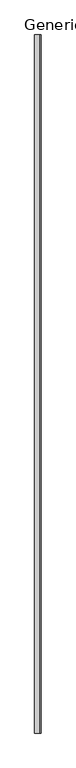
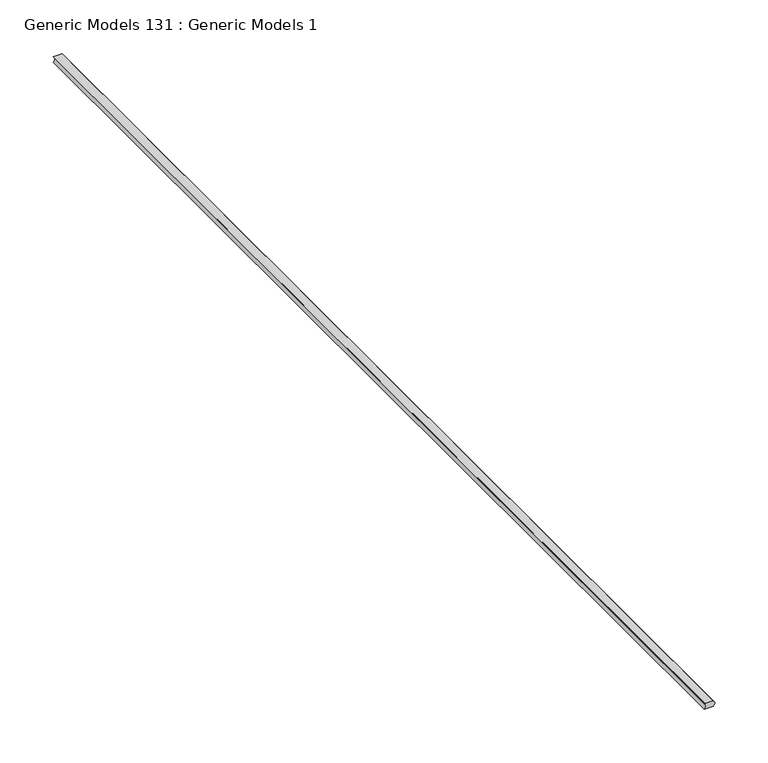
"""IFC4 building model written with IfcOpenShell, lengths in millimetres: proxy geometry, Generic Models 131 : Generic Models 1."""

from ifc_helpers import new_model, si_unit, point, frame, frame_2d, origin, place, context, project, spatial, polyline, circle_curve, trimmed, segment, composite_curve, outline, extrude, source, transform, mapped, element, save


def generic_models_131_generic_models_1_f9918aae(model_context):
    return source(origin(), model_context, "Body", "SweptSolid", [
        extrude(outline(composite_curve([segment(polyline([(0.0, 50777.775), (0.0, 50787.3)]), True, "CONTINUOUS"), segment(trimmed(circle_curve(frame_2d((3.175, 50784.3852595)), 4.3100275), [point((0.0, 50787.3))], [point((6.35, 50787.3))], False, "CARTESIAN"), True, "CONTINUOUS"), segment(polyline([(6.35, 50787.3), (6.35, 50777.775)]), True, "CONTINUOUS"), segment(trimmed(circle_curve(frame_2d((3.175, 50774.8602595)), 4.3100275), [point((6.35, 50777.775))], [point((0.0, 50777.775))], True, "CARTESIAN"), True, "CONTINUOUS")], self_intersect=False)), frame((0.0, 0.0, 0.0), z_axis=(0.0, 1.0, 0.0), x_axis=(0.0, 0.0, 1.0)), (0.0, 0.0, 1.0), 1219.2),
    ])


if __name__ == "__main__":
    model = new_model("IFC4")
    model_context = context("Model", 3, world=origin())
    ifc_project = project(units=[si_unit("LENGTHUNIT", "METRE", prefix="MILLI")], contexts=[model_context])
    site = spatial("IfcSite", under=ifc_project)
    building = spatial("IfcBuilding", under=site)
    placement = place(None, origin())
    generic_models_131_generic_models_1_shape = generic_models_131_generic_models_1_f9918aae(model_context)
    element("IfcBuildingElementProxy", 1, Name="Generic Models 131 : Generic Models 1", ObjectType="Generic Models 131 : Generic Models 1", at=placement, inside=building, context=model_context, shape_type="MappedRepresentation", body=[
        mapped(generic_models_131_generic_models_1_shape, transform((0.0, 0.0, 0.0), x_axis=(1.0, 0.0, 0.0), y_axis=(0.0, 1.0, 0.0), z_axis=(0.0, 0.0, 1.0))),
    ])
    save(model, "model.ifc")

# Revit data of these elements
# Element 1 (IfcBuildingElementProxy, "Generic Models 131 : Generic Models 1")
#   Materials on its faces: "ACOUSTICAL SEALANT"
# Materials
#   "ACOUSTICAL SEALANT": class "Unassigned", colour RGB 120 120 120, transparency 0, Cost = 0
